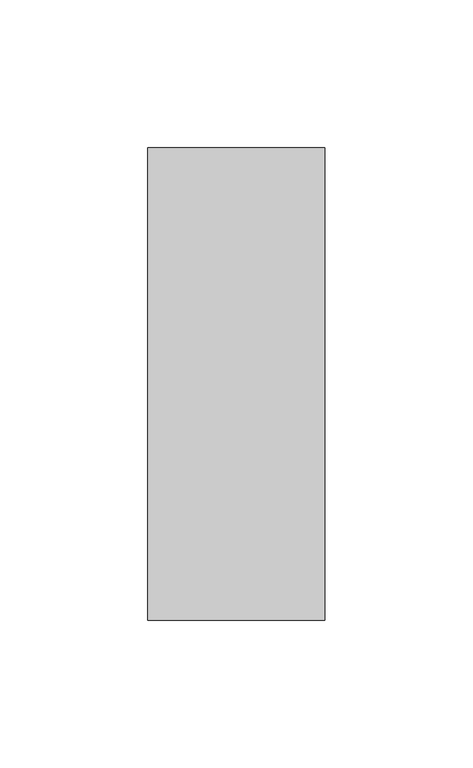
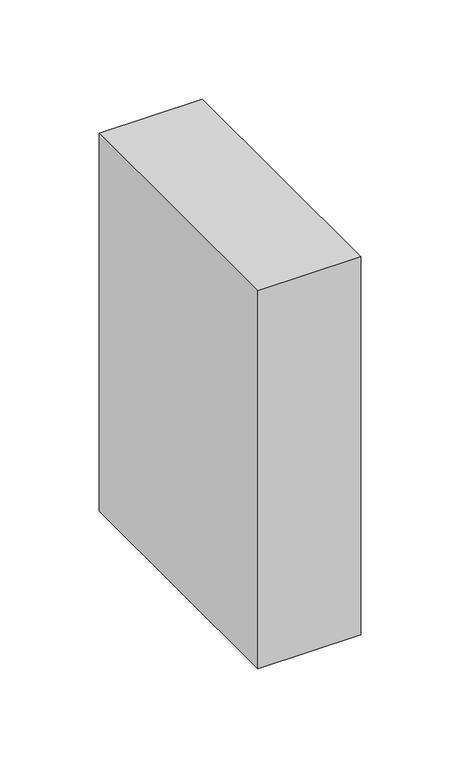
"""IFC4 building model written with IfcOpenShell, lengths in millimetres: column geometry, Madeira de lei-Coluna : Pontalete 6X16cm."""

from ifc_helpers import new_model, si_unit, frame, origin, place, context, project, spatial, polyline, outline, extrude, source, transform, mapped, element, save


def column_6cc9e01b(model_context):
    return source(origin(), model_context, "Body", "SweptSolid", [
        extrude(outline(polyline([(30.0, 80.0), (30.0, -80.0), (-30.0, -80.0), (-30.0, 80.0), (30.0, 80.0)])), frame((0.0, 0.0, 4460.0), z_axis=(0.0, 0.0, 1.0), x_axis=(1.0, 0.0, 0.0)), (0.0, 0.0, 1.0), 233.0),
    ])


if __name__ == "__main__":
    model = new_model("IFC4")
    model_context = context("Model", 3, world=origin())
    ifc_project = project(units=[si_unit("LENGTHUNIT", "METRE", prefix="MILLI")], contexts=[model_context])
    site = spatial("IfcSite", under=ifc_project)
    building = spatial("IfcBuilding", under=site)
    placement = place(None, origin())
    column_shape = column_6cc9e01b(model_context)
    element("IfcColumn", 1, ObjectType="Madeira de lei-Coluna : Pontalete 6X16cm", at=placement, inside=building, context=model_context, shape_type="MappedRepresentation", body=[
        mapped(column_shape, transform((0.0, 0.0, 0.0), x_axis=(1.0, 0.0, 0.0), y_axis=(0.0, 1.0, 0.0), z_axis=(0.0, 0.0, 1.0))),
    ])
    save(model, "model.ifc")

# Revit data of these elements
# Type "Madeira de lei-Coluna : Pontalete 6X16cm"
#   A = 0.01952 m²
#   b = 0.06 m
#   d = 0.16 m
#   Structural Material [instance default] = none
#   Assembly Code = ""
# Element 1 (IfcColumn, "Madeira de lei-Coluna : Pontalete 6X16cm")
#   Structural Material = .MADEIRAMENTO
#   Materials on its faces: ".MADEIRAMENTO"
# Materials
#   ".MADEIRAMENTO": class ".CC_MADEIRAS", colour RGB 212 179 113, transparency 0, Cost = 0
